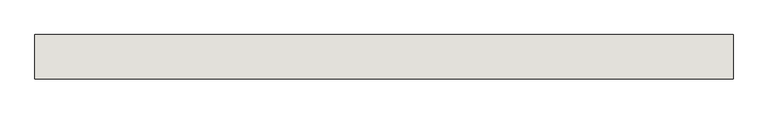
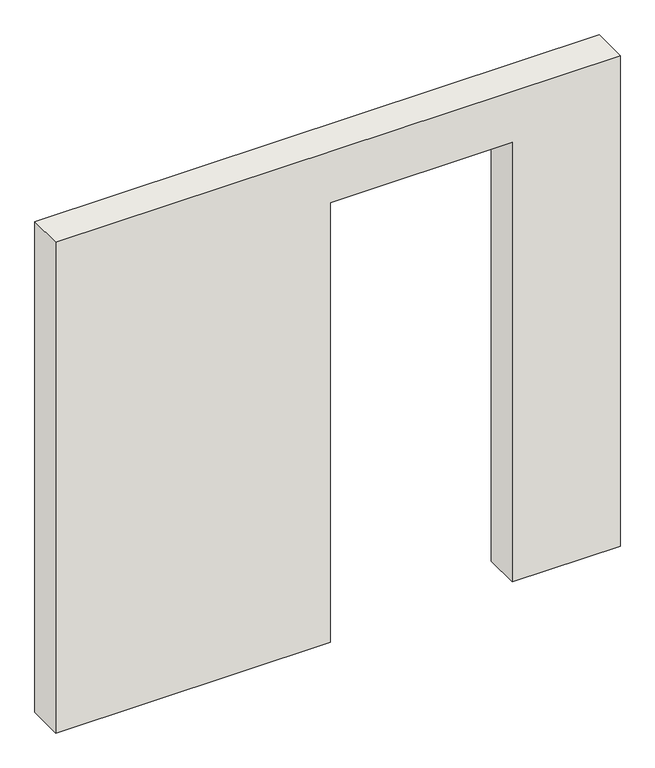
"""IFC4 building model written with IfcOpenShell, lengths in millimetres: wall geometry, 0_3d_modell."""

from ifc_helpers import new_model, si_unit, frame, origin, place, context, project, spatial, polyline, outline, extrude, source, transform, mapped, element, save


def wall_4e7b00e6(model_context):
    return source(origin(), model_context, "Body", "SweptSolid", [
        extrude(outline(polyline([(2580.0, 2534.0204176), (0.0, 2534.0204176), (0.0, 3133.4), (2880.0, 3133.4), (2880.0, 0.0), (0.0, 0.0), (0.0, 1524.0204176), (2580.0, 1524.0204176), (2580.0, 2534.0204176)])), frame((0.0, 0.0, 0.0), z_axis=(0.0, 1.0, 0.0), x_axis=(0.0, 0.0, 1.0)), (0.0, 0.0, 1.0), 200.0),
    ])


if __name__ == "__main__":
    model = new_model("IFC4")
    model_context = context("Model", 3, world=origin())
    ifc_project = project(units=[si_unit("LENGTHUNIT", "METRE", prefix="MILLI")], contexts=[model_context])
    site = spatial("IfcSite", under=ifc_project)
    building = spatial("IfcBuilding", under=site)
    placement = place(None, origin())
    wall_shape = wall_4e7b00e6(model_context)
    element("IfcWall", 1, ObjectType="0_3d_modell", at=placement, inside=building, context=model_context, shape_type="MappedRepresentation", body=[
        mapped(wall_shape, transform((0.0, 0.0, 0.0), x_axis=(1.0, 0.0, 0.0), y_axis=(0.0, 1.0, 0.0), z_axis=(0.0, 0.0, 1.0))),
    ])
    save(model, "model.ifc")

# Revit data of these elements
# Element 1 (IfcWall, "0_3d_modell")
#   Materials on its faces: "material wardrobe b 1"
# Materials
#   "material wardrobe b 1": class "Unassigned", colour RGB 128 128 128, transparency 0
